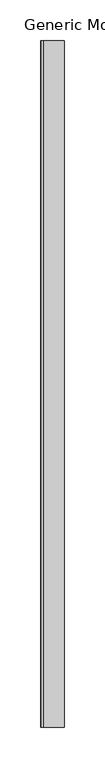
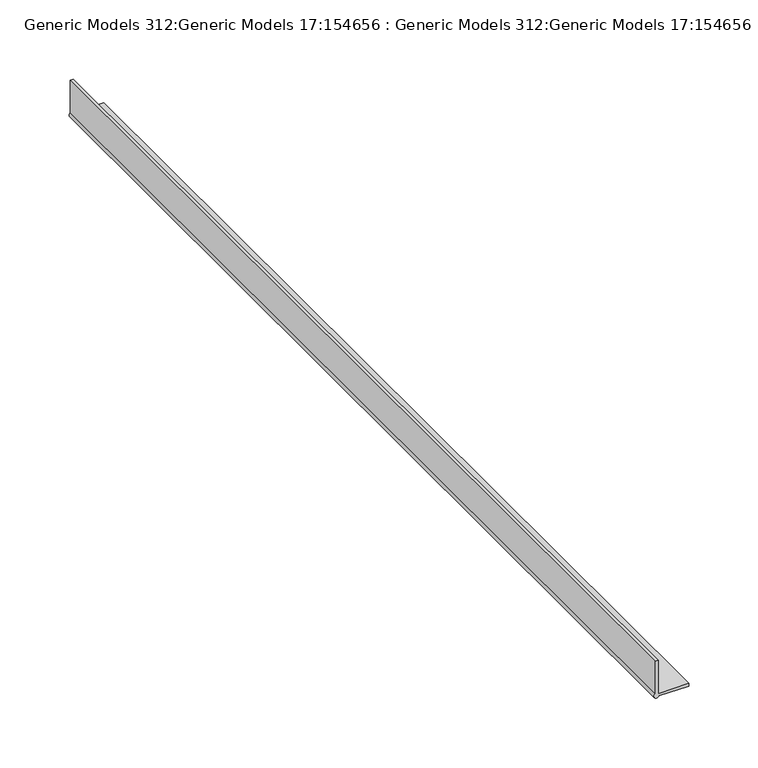
"""IFC4 building model written with IfcOpenShell, lengths in millimetres: proxy geometry, Generic Models 312:Generic Models 17:154656 : Generic Models 312:Generic Models 17:154656."""

from ifc_helpers import new_model, si_unit, point, frame, frame_2d, origin, place, context, project, spatial, polyline, circle_curve, trimmed, segment, composite_curve, outline, extrude, source, transform, mapped, element, save


def generic_models_312_generic_models_17_154656_generic_models_09943ed6(model_context):
    return source(origin(), model_context, "Body", "SweptSolid", [
        extrude(outline(composite_curve([segment(trimmed(circle_curve(frame_2d((2948.1270275, 1421.4076917)), 2.1956516), [point((2949.9575447, 1420.1952178))], [point((2947.1300253, 1423.3639312))], False, "CARTESIAN"), True, "CONTINUOUS"), segment(polyline([(2947.1300253, 1423.3639312), (2947.1300253, 1448.2058187), (2949.3759659, 1448.2058187), (2949.3759659, 1422.6399618), (2978.8800253, 1422.6399618), (2978.8800253, 1420.1952178), (2949.9575447, 1420.1952178)]), True, "CONTINUOUS")], self_intersect=False)), frame((0.0, 4097.6531132, 0.0), z_axis=(0.0, 1.0, 0.0), x_axis=(0.0, 0.0, 1.0)), (0.0, 0.0, 1.0), 846.0415953),
    ])


if __name__ == "__main__":
    model = new_model("IFC4")
    model_context = context("Model", 3, world=origin())
    ifc_project = project(units=[si_unit("LENGTHUNIT", "METRE", prefix="MILLI")], contexts=[model_context])
    site = spatial("IfcSite", under=ifc_project)
    building = spatial("IfcBuilding", under=site)
    placement = place(None, origin())
    generic_models_312_generic_models_17_154656_generic_models_shape = generic_models_312_generic_models_17_154656_generic_models_09943ed6(model_context)
    element("IfcBuildingElementProxy", 1, Name="Generic Models 312:Generic Models 17:154656 : Generic Models 312:Generic Models 17:154656", ObjectType="Generic Models 312:Generic Models 17:154656 : Generic Models 312:Generic Models 17:154656", at=placement, inside=building, context=model_context, shape_type="MappedRepresentation", body=[
        mapped(generic_models_312_generic_models_17_154656_generic_models_shape, transform((0.0, 0.0, 0.0), x_axis=(1.0, 0.0, 0.0), y_axis=(0.0, 1.0, 0.0), z_axis=(0.0, 0.0, 1.0))),
    ])
    save(model, "model.ifc")

# Revit data of these elements
# Type "Generic Models 312:Generic Models 17:154656 : Generic Models 312:Generic Models 17:154656"
#   NameOverride = "Generic Models 312:Generic Models 17:154656"
#   ObjectTypeOverride = "Generic Models 312:Generic Models 17"
#   Reference = "Generic Models 17"
#   Category = "Generic Models"
#   Tag = "154656"
# Element 1 (IfcBuildingElementProxy, "Generic Models 312:Generic Models 17:154656 : Generic Models 312:Generic Models 17:154656")
#   Materials on its faces: "_DRYWALL CORNER BEAD 25414"
# Materials
#   "_DRYWALL CORNER BEAD 25414": class "Unassigned", colour RGB 253 192 103, transparency 0
